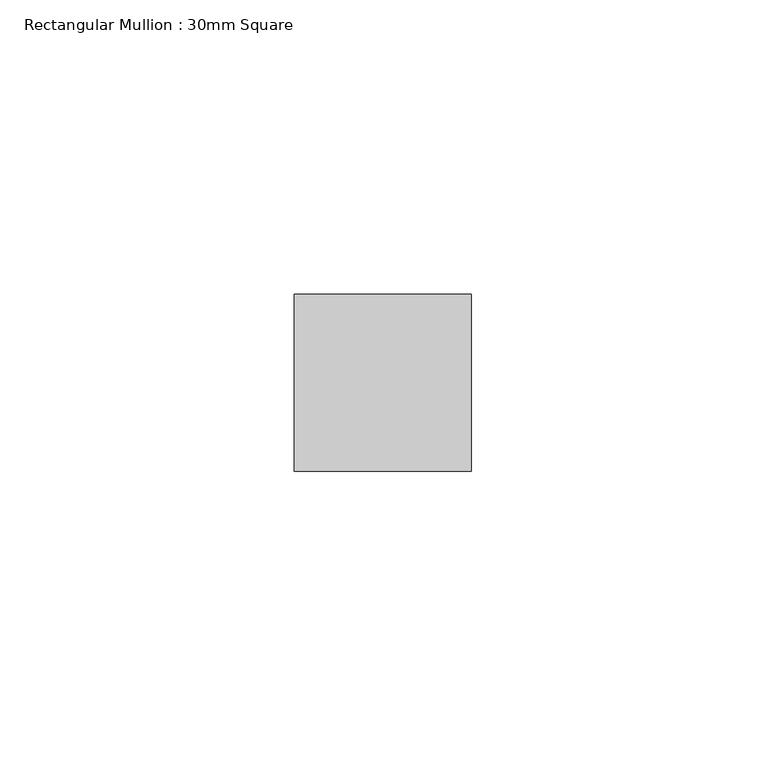
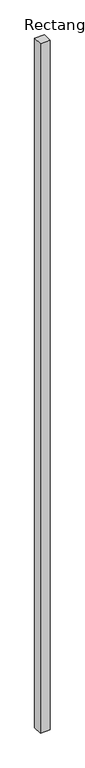
"""IFC4 building model written with IfcOpenShell, lengths in millimetres: member geometry, Rectangular Mullion : 30mm Square."""

import ifcopenshell
import ifcopenshell.guid

model = None  # the IFC model being written
_history = None  # IfcOwnerHistory: only IFC2X3 demands one
_inside = {}  # id of a spatial element -> (the spatial element, [elements in it])
_under = {}  # id of a project, library or spatial element -> (it, [spatial elements below it])
_declared = {}  # id of a project -> (the project, [libraries it declares])
_typed = {}  # id of a type object -> (the type object, [elements of that type])
_made_of = {}  # id of a material, layer set ... -> (it, [elements and type objects made of it])


def new_model(schema):
    """Start an empty IFC model of exactly this schema.

    Asked for "IFC4X3", IfcOpenShell would pick the latest addendum, in which some entities
    have other attributes; the version numbers below select the first issue.
    IFC2X3 requires an IfcOwnerHistory on every rooted entity: one is made here for all.
    """
    global model, _history
    if schema == "IFC4X3":
        model = ifcopenshell.file(schema_version=(4, 3, 0, 0))
    else:
        model = ifcopenshell.file(schema=schema)
    _inside.clear()
    _under.clear()
    _declared.clear()
    _typed.clear()
    _made_of.clear()
    _history = None
    if model.schema == "IFC2X3":
        org = make("IfcOrganization", Name="unknown")
        user = make(
            "IfcPersonAndOrganization",
            ThePerson=make("IfcPerson", FamilyName="unknown"),
            TheOrganization=org,
        )
        app = make(
            "IfcApplication",
            ApplicationDeveloper=org,
            Version="unknown",
            ApplicationFullName="unknown",
            ApplicationIdentifier="unknown",
        )
        _history = make(
            "IfcOwnerHistory",
            OwningUser=user,
            OwningApplication=app,
            ChangeAction="ADDED",
            CreationDate=0,
        )
    return model


def make(cls, **values):
    """One entity of the class cls with the attributes given. An attribute that is None is left unset."""
    return model.create_entity(
        cls, **{name: value for name, value in values.items() if value is not None}
    )


def rooted(cls, **values):
    """An entity with a GlobalId (a new one), such as an element, a storey or a relation."""
    return make(cls, GlobalId=ifcopenshell.guid.new(), OwnerHistory=_history, **values)


def si_unit(unit_type, name, prefix=None):
    """IfcSIUnit, for example si_unit("LENGTHUNIT", "METRE", prefix="MILLI")."""
    return make("IfcSIUnit", UnitType=unit_type, Prefix=prefix, Name=name)


def assignment(units):
    """IfcUnitAssignment: the units of a project."""
    return None if units is None else make("IfcUnitAssignment", Units=units)


def point(xyz):
    """IfcCartesianPoint."""
    return None if xyz is None else make("IfcCartesianPoint", Coordinates=xyz)


def direction(xyz):
    """IfcDirection."""
    return None if xyz is None else make("IfcDirection", DirectionRatios=xyz)


def frame(location, z_axis=None, x_axis=None):
    """IfcAxis2Placement3D, a coordinate frame: its origin and axes. An axis left out is left unset."""
    return make(
        "IfcAxis2Placement3D",
        Location=point(location),
        Axis=direction(z_axis),
        RefDirection=direction(x_axis),
    )


def origin():
    """The frame at (0, 0, 0) with its axes left unset."""
    return frame((0.0, 0.0, 0.0))


def place(relative_to, where):
    """IfcLocalPlacement: puts the frame where relative to a parent placement (None: the world)."""
    return make(
        "IfcLocalPlacement", PlacementRelTo=relative_to, RelativePlacement=where
    )


def context(
    kind, dimensions, precision=None, world=None, true_north=None, identifier=None
):
    """IfcGeometricRepresentationContext, for example the 3D "Model" context."""
    return make(
        "IfcGeometricRepresentationContext",
        ContextIdentifier=identifier,
        ContextType=kind,
        CoordinateSpaceDimension=dimensions,
        Precision=precision,
        WorldCoordinateSystem=world,
        TrueNorth=true_north,
    )


def project(units=None, contexts=None):
    """IfcProject with its units and contexts."""
    return rooted(
        "IfcProject",
        Name="project",
        RepresentationContexts=contexts,
        UnitsInContext=assignment(units),
    )


def spatial(cls, under=None, at=None, **own):
    """A site, building, storey or space (cls), placed at a placement, below another one or the project."""
    s = rooted(cls, ObjectPlacement=at, **own)
    if under is not None:
        _under.setdefault(under.id(), (under, []))[1].append(s)
    return s


def polyline(points):
    """IfcPolyline through the points."""
    return make("IfcPolyline", Points=[point(p) for p in points])


def outline(outer, holes=None, kind="AREA"):
    """IfcArbitraryClosedProfileDef: a profile drawn as a closed curve; with holes, ...WithVoids."""
    if holes is None:
        return make("IfcArbitraryClosedProfileDef", ProfileType=kind, OuterCurve=outer)
    return make(
        "IfcArbitraryProfileDefWithVoids",
        ProfileType=kind,
        OuterCurve=outer,
        InnerCurves=holes,
    )


def extrude(swept, where, along, depth):
    """IfcExtrudedAreaSolid: the profile swept, set in the frame where, extruded along a direction by depth."""
    return make(
        "IfcExtrudedAreaSolid",
        SweptArea=swept,
        Position=where,
        ExtrudedDirection=direction(along),
        Depth=depth,
    )


def shape(context_of_items, identifier, shape_type, items):
    """IfcShapeRepresentation: the items that make up one representation, for example the "Body"."""
    return make(
        "IfcShapeRepresentation",
        ContextOfItems=context_of_items,
        RepresentationIdentifier=identifier,
        RepresentationType=shape_type,
        Items=items,
    )


def source(mapping_origin, context_of_items, identifier, shape_type, items):
    """IfcRepresentationMap: a shape defined once, which mapped items show again and again."""
    return make(
        "IfcRepresentationMap",
        MappingOrigin=mapping_origin,
        MappedRepresentation=shape(context_of_items, identifier, shape_type, items),
    )


def transform(
    local_origin,
    x_axis=None,
    y_axis=None,
    z_axis=None,
    scale=None,
    scale2=None,
    scale3=None,
    uniform=True,
):
    """IfcCartesianTransformationOperator3D, or its non-uniform kind. x_axis, y_axis, z_axis: its Axis1, 2, 3."""
    if uniform:
        return make(
            "IfcCartesianTransformationOperator3D",
            Axis1=direction(x_axis),
            Axis2=direction(y_axis),
            LocalOrigin=point(local_origin),
            Scale=scale,
            Axis3=direction(z_axis),
        )
    return make(
        "IfcCartesianTransformationOperator3DnonUniform",
        Axis1=direction(x_axis),
        Axis2=direction(y_axis),
        LocalOrigin=point(local_origin),
        Scale=scale,
        Axis3=direction(z_axis),
        Scale2=scale2,
        Scale3=scale3,
    )


def mapped(mapping_source, mapping_target):
    """IfcMappedItem: shows the shape of a source again, moved by a transform."""
    return make(
        "IfcMappedItem", MappingSource=mapping_source, MappingTarget=mapping_target
    )


def made_of(thing, what):
    """Note that an element or type object is made of a material, layer set ...; save() writes the relation."""
    if what is not None:
        _made_of.setdefault(what.id(), (what, []))[1].append(thing)
    return thing


def element(
    cls,
    number,
    at=None,
    inside=None,
    cuts=None,
    type_object=None,
    material=None,
    context=None,
    identifier="Body",
    shape_type=None,
    held_by="IfcProductDefinitionShape",
    body=None,
    shapes=None,
    **own,
):
    """One element of the class cls, such as IfcWall. Its Tag is "e" and its number.

    at: its placement. inside: the storey or other place that contains it. cuts: it is an
    opening in that element (IfcRelVoidsElement). A single representation is given by context,
    identifier, shape_type and body (its items); several are given by shapes. held_by: the class
    of the entity that holds the representations. save() writes the other relations.
    """
    e = rooted(cls, Tag="e%d" % number, ObjectPlacement=at, **own)
    if body is not None:
        shapes = [shape(context, identifier, shape_type, body)]
    if shapes is not None:
        e.Representation = make(held_by, Representations=shapes)
    if inside is not None:
        _inside.setdefault(inside.id(), (inside, []))[1].append(e)
    if cuts is not None:
        rooted(
            "IfcRelVoidsElement", RelatingBuildingElement=cuts, RelatedOpeningElement=e
        )
    if type_object is not None:
        _typed.setdefault(type_object.id(), (type_object, []))[1].append(e)
    return made_of(e, material)


def aggregate(whole, parts):
    """IfcRelAggregates: a whole, such as a stair, and the parts it consists of."""
    return rooted("IfcRelAggregates", RelatingObject=whole, RelatedObjects=parts)


def save(model, path):
    """Write the relations noted so far, then the file.

    IfcRelAggregates (storeys below a building ...), IfcRelContainedInSpatialStructure (elements
    in a storey), IfcRelDefinesByType, IfcRelAssociatesMaterial and IfcRelDeclares: one each for
    every whole, place, type object, material and project.
    """
    for whole, parts in _under.values():
        aggregate(whole, parts)
    for where, things in _inside.values():
        rooted(
            "IfcRelContainedInSpatialStructure",
            RelatedElements=things,
            RelatingStructure=where,
        )
    for kind, things in _typed.values():
        rooted("IfcRelDefinesByType", RelatedObjects=things, RelatingType=kind)
    for what, things in _made_of.values():
        rooted("IfcRelAssociatesMaterial", RelatedObjects=things, RelatingMaterial=what)
    for by, libraries in _declared.values():
        rooted("IfcRelDeclares", RelatingContext=by, RelatedDefinitions=libraries)
    model.write(path)


def rectangular_mullion_30mm_square_eb36dfb5(model_context):
    return source(origin(), model_context, "Body", "SweptSolid", [
        extrude(outline(polyline([(15.0, 15.0), (15.0, -15.0), (-15.0, -15.0), (-15.0, 15.0), (15.0, 15.0)])), frame((0.0, 0.0, -2243.3891851), z_axis=(0.0, 0.0, 1.0), x_axis=(1.0, 0.0, 0.0)), (0.0, 0.0, 1.0), 2243.3891851),
    ])


if __name__ == "__main__":
    model = new_model("IFC4")
    model_context = context("Model", 3, world=origin())
    ifc_project = project(units=[si_unit("LENGTHUNIT", "METRE", prefix="MILLI")], contexts=[model_context])
    site = spatial("IfcSite", under=ifc_project)
    building = spatial("IfcBuilding", under=site)
    placement = place(None, origin())
    rectangular_mullion_30mm_square_shape = rectangular_mullion_30mm_square_eb36dfb5(model_context)
    element("IfcMember", 1, ObjectType="Rectangular Mullion : 30mm Square", at=placement, inside=building, context=model_context, shape_type="MappedRepresentation", body=[
        mapped(rectangular_mullion_30mm_square_shape, transform((0.0, 0.0, 0.0), x_axis=(1.0, 0.0, 0.0), y_axis=(0.0, 1.0, 0.0), z_axis=(0.0, 0.0, 1.0))),
    ])
    save(model, "model.ifc")

# Revit data of these elements
# Type "Rectangular Mullion : 30mm Square"
#   built-in parameter 1007304 = 0.0984252 (stored number, unit not read)
#   built-in parameter 1007301 = 0.0492126 (stored number, unit not read)
#   built-in parameter 1007300 = 0.0492126 (stored number, unit not read)
# Element 1 (IfcMember, "Rectangular Mullion : 30mm Square")
#   Materials on its faces: "Aluminum"
# Materials
#   "Aluminum": class "Metal", colour RGB 244 244 244, transparency 0, Description = "Aluminum 6061", Cost = 0
